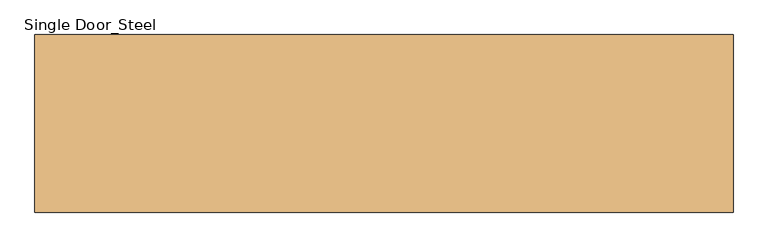
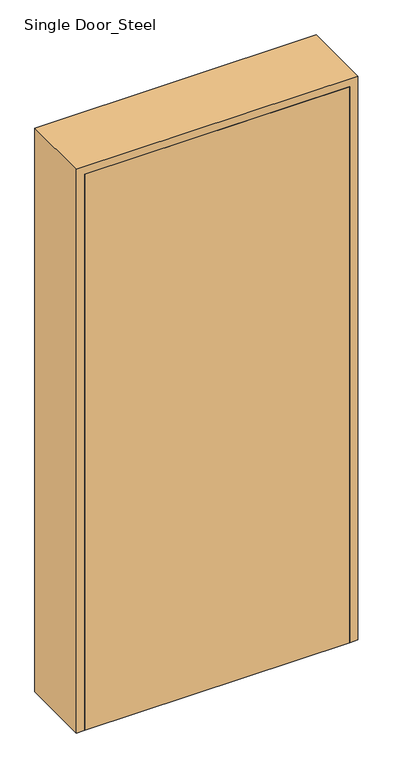
"""IFC4 building model written with IfcOpenShell, lengths in millimetres: door geometry, Single Door_Steel : H_DR_AR B12_Door_Single FSD 01."""

from ifc_helpers import new_model, si_unit, origin, origin_with_axes, place, context, project, spatial, polyline, outline, extrude, faceted_brep, source, transform, mapped, element, save


def single_door_steel_f73fbc53(model_context):
    return source(origin(), model_context, "Body", "SolidModel", [
        extrude(outline(polyline([(480.0, -130.0), (-480.0, -130.0), (-480.0, -95.0), (480.0, -95.0), (480.0, -130.0)])), origin_with_axes(), (0.0, 0.0, 1.0), 2130.0),
        faceted_brep([(480.0, -130.0, 0.0), (480.0, -95.0, 0.0), (460.0, -95.0, 0.0), (460.0, 95.0, 0.0), (480.0, 95.0, 0.0), (480.0, 130.0, 0.0), (510.0, 130.0, 0.0), (510.0, -130.0, 0.0), (510.0, -130.0, 2160.0), (-510.0, -130.0, 2160.0), (-510.0, -130.0, 0.0), (-480.0, -130.0, 0.0), (-480.0, -130.0, 2130.0), (480.0, -130.0, 2130.0), (510.0, 130.0, 2160.0), (480.0, 130.0, 2130.0), (-480.0, 130.0, 2130.0), (-480.0, 130.0, 0.0), (-510.0, 130.0, 0.0), (-510.0, 130.0, 2160.0), (480.0, 95.0, 2130.0), (460.0, 95.0, 2110.0), (-460.0, 95.0, 2110.0), (-460.0, 95.0, 0.0), (-480.0, 95.0, 0.0), (-480.0, 95.0, 2130.0), (460.0, -95.0, 2110.0), (480.0, -95.0, 2130.0), (-480.0, -95.0, 2130.0), (-480.0, -95.0, 0.0), (-460.0, -95.0, 0.0), (-460.0, -95.0, 2110.0)], [[[0, 1, 2, 3, 4, 5, 6, 7]], [[7, 8, 9, 10, 11, 12, 13, 0]], [[6, 14, 8, 7]], [[5, 15, 16, 17, 18, 19, 14, 6]], [[4, 20, 15, 5]], [[3, 21, 22, 23, 24, 25, 20, 4]], [[2, 26, 21, 3]], [[1, 27, 28, 29, 30, 31, 26, 2]], [[0, 13, 27, 1]], [[12, 11, 29, 28]], [[11, 10, 18, 17, 24, 23, 30, 29]], [[19, 18, 10, 9]], [[25, 24, 17, 16]], [[31, 30, 23, 22]], [[14, 19, 9, 8]], [[20, 25, 16, 15]], [[26, 31, 22, 21]], [[13, 12, 28, 27]]]),
    ])


if __name__ == "__main__":
    model = new_model("IFC4")
    model_context = context("Model", 3, world=origin())
    ifc_project = project(units=[si_unit("LENGTHUNIT", "METRE", prefix="MILLI")], contexts=[model_context])
    site = spatial("IfcSite", under=ifc_project)
    building = spatial("IfcBuilding", under=site)
    placement = place(None, origin())
    single_door_steel_shape = single_door_steel_f73fbc53(model_context)
    element("IfcDoor", 1, ObjectType="Single Door_Steel : H_DR_AR B12_Door_Single FSD 01", at=placement, inside=building, context=model_context, shape_type="MappedRepresentation", body=[
        mapped(single_door_steel_shape, transform((0.0, 0.0, 0.0), x_axis=(1.0, 0.0, 0.0), y_axis=(0.0, 1.0, 0.0), z_axis=(0.0, 0.0, 1.0))),
    ])
    save(model, "model.ifc")

# Revit data of these elements
# Type "Single Door_Steel : H_DR_AR B12_Door_Single FSD 01"
#   Type Mark = "FRD"
#   Analytic Construction = "<None>"
#   프레임 투영 외부. = 25 mm
#   프레임 투영 내부. = 25 mm
#   프레임 폭 = 75 mm
#   Height = 2160 mm
#   Width = 1020 mm
#   Define Thermal Properties by = 1
#   문 패널 = none
#   문 프레임 = none
#   Function = (empty or 0)
#   Wall Closure = (empty or 0)
